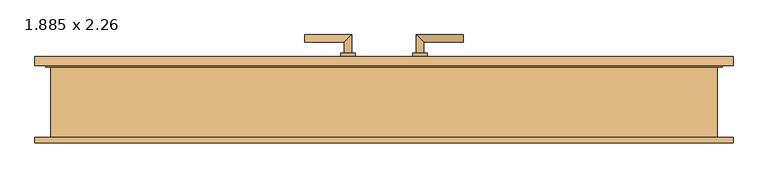
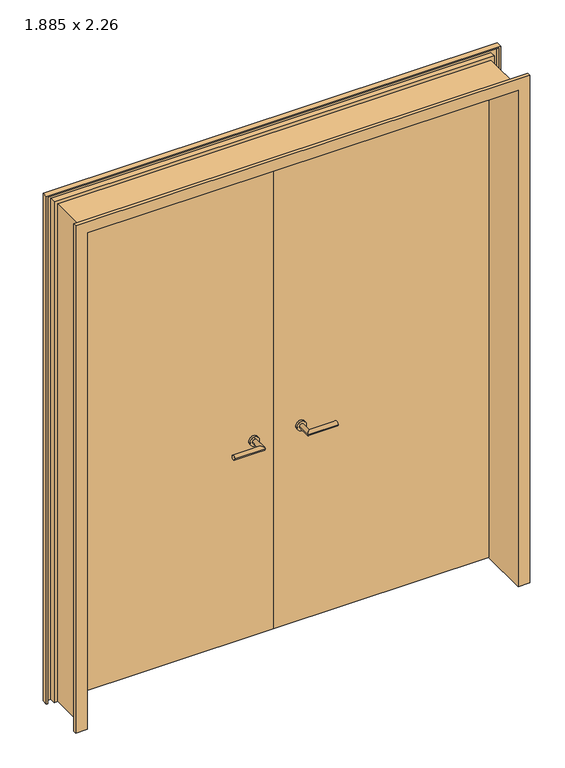
"""IFC4 building model written with IfcOpenShell, lengths in millimetres: door geometry, Drehflügel 2-flg - Stahlzarge : 1.885 x 2.26."""

import ifcopenshell
import ifcopenshell.guid

model = None  # the IFC model being written
_history = None  # IfcOwnerHistory: only IFC2X3 demands one
_inside = {}  # id of a spatial element -> (the spatial element, [elements in it])
_under = {}  # id of a project, library or spatial element -> (it, [spatial elements below it])
_declared = {}  # id of a project -> (the project, [libraries it declares])
_typed = {}  # id of a type object -> (the type object, [elements of that type])
_made_of = {}  # id of a material, layer set ... -> (it, [elements and type objects made of it])


def new_model(schema):
    """Start an empty IFC model of exactly this schema.

    Asked for "IFC4X3", IfcOpenShell would pick the latest addendum, in which some entities
    have other attributes; the version numbers below select the first issue.
    IFC2X3 requires an IfcOwnerHistory on every rooted entity: one is made here for all.
    """
    global model, _history
    if schema == "IFC4X3":
        model = ifcopenshell.file(schema_version=(4, 3, 0, 0))
    else:
        model = ifcopenshell.file(schema=schema)
    _inside.clear()
    _under.clear()
    _declared.clear()
    _typed.clear()
    _made_of.clear()
    _history = None
    if model.schema == "IFC2X3":
        org = make("IfcOrganization", Name="unknown")
        user = make(
            "IfcPersonAndOrganization",
            ThePerson=make("IfcPerson", FamilyName="unknown"),
            TheOrganization=org,
        )
        app = make(
            "IfcApplication",
            ApplicationDeveloper=org,
            Version="unknown",
            ApplicationFullName="unknown",
            ApplicationIdentifier="unknown",
        )
        _history = make(
            "IfcOwnerHistory",
            OwningUser=user,
            OwningApplication=app,
            ChangeAction="ADDED",
            CreationDate=0,
        )
    return model


def make(cls, **values):
    """One entity of the class cls with the attributes given. An attribute that is None is left unset."""
    return model.create_entity(
        cls, **{name: value for name, value in values.items() if value is not None}
    )


def rooted(cls, **values):
    """An entity with a GlobalId (a new one), such as an element, a storey or a relation."""
    return make(cls, GlobalId=ifcopenshell.guid.new(), OwnerHistory=_history, **values)


def si_unit(unit_type, name, prefix=None):
    """IfcSIUnit, for example si_unit("LENGTHUNIT", "METRE", prefix="MILLI")."""
    return make("IfcSIUnit", UnitType=unit_type, Prefix=prefix, Name=name)


def assignment(units):
    """IfcUnitAssignment: the units of a project."""
    return None if units is None else make("IfcUnitAssignment", Units=units)


def point(xyz):
    """IfcCartesianPoint."""
    return None if xyz is None else make("IfcCartesianPoint", Coordinates=xyz)


def direction(xyz):
    """IfcDirection."""
    return None if xyz is None else make("IfcDirection", DirectionRatios=xyz)


def frame(location, z_axis=None, x_axis=None):
    """IfcAxis2Placement3D, a coordinate frame: its origin and axes. An axis left out is left unset."""
    return make(
        "IfcAxis2Placement3D",
        Location=point(location),
        Axis=direction(z_axis),
        RefDirection=direction(x_axis),
    )


def frame_2d(location, x_axis=None):
    """IfcAxis2Placement2D, a coordinate frame in the plane: its origin and x axis."""
    return make(
        "IfcAxis2Placement2D", Location=point(location), RefDirection=direction(x_axis)
    )


def origin():
    """The frame at (0, 0, 0) with its axes left unset."""
    return frame((0.0, 0.0, 0.0))


def origin_with_axes():
    """The frame at (0, 0, 0) with the z axis (0, 0, 1) and the x axis (1, 0, 0) written out."""
    return frame((0.0, 0.0, 0.0), z_axis=(0.0, 0.0, 1.0), x_axis=(1.0, 0.0, 0.0))


def place(relative_to, where):
    """IfcLocalPlacement: puts the frame where relative to a parent placement (None: the world)."""
    return make(
        "IfcLocalPlacement", PlacementRelTo=relative_to, RelativePlacement=where
    )


def context(
    kind, dimensions, precision=None, world=None, true_north=None, identifier=None
):
    """IfcGeometricRepresentationContext, for example the 3D "Model" context."""
    return make(
        "IfcGeometricRepresentationContext",
        ContextIdentifier=identifier,
        ContextType=kind,
        CoordinateSpaceDimension=dimensions,
        Precision=precision,
        WorldCoordinateSystem=world,
        TrueNorth=true_north,
    )


def project(units=None, contexts=None):
    """IfcProject with its units and contexts."""
    return rooted(
        "IfcProject",
        Name="project",
        RepresentationContexts=contexts,
        UnitsInContext=assignment(units),
    )


def spatial(cls, under=None, at=None, **own):
    """A site, building, storey or space (cls), placed at a placement, below another one or the project."""
    s = rooted(cls, ObjectPlacement=at, **own)
    if under is not None:
        _under.setdefault(under.id(), (under, []))[1].append(s)
    return s


def polyline(points):
    """IfcPolyline through the points."""
    return make("IfcPolyline", Points=[point(p) for p in points])


def circle_curve(where, radius):
    """IfcCircle in the frame where."""
    return make("IfcCircle", Position=where, Radius=radius)


def ellipse_curve(where, semi_axis1, semi_axis2):
    """IfcEllipse in the frame where."""
    return make(
        "IfcEllipse", Position=where, SemiAxis1=semi_axis1, SemiAxis2=semi_axis2
    )


def trimmed(basis, trim1, trim2, sense, master):
    """IfcTrimmedCurve: the piece of a basis curve between two trims."""
    return make(
        "IfcTrimmedCurve",
        BasisCurve=basis,
        Trim1=trim1,
        Trim2=trim2,
        SenseAgreement=sense,
        MasterRepresentation=master,
    )


def segment(curve, same_sense, transition):
    """IfcCompositeCurveSegment."""
    return make(
        "IfcCompositeCurveSegment",
        Transition=transition,
        SameSense=same_sense,
        ParentCurve=curve,
    )


def composite_curve(segments, self_intersect=None):
    """IfcCompositeCurve: segments joined end to end."""
    return make("IfcCompositeCurve", Segments=segments, SelfIntersect=self_intersect)


def outline(outer, holes=None, kind="AREA"):
    """IfcArbitraryClosedProfileDef: a profile drawn as a closed curve; with holes, ...WithVoids."""
    if holes is None:
        return make("IfcArbitraryClosedProfileDef", ProfileType=kind, OuterCurve=outer)
    return make(
        "IfcArbitraryProfileDefWithVoids",
        ProfileType=kind,
        OuterCurve=outer,
        InnerCurves=holes,
    )


def extrude(swept, where, along, depth):
    """IfcExtrudedAreaSolid: the profile swept, set in the frame where, extruded along a direction by depth."""
    return make(
        "IfcExtrudedAreaSolid",
        SweptArea=swept,
        Position=where,
        ExtrudedDirection=direction(along),
        Depth=depth,
    )


def faces_of(points, faces, orient=None, outer=None):
    """IfcFace entities. A face is a list of loops; a loop is a list of indices into points, from 0.

    orient and outer hold one flag for each loop. By default every Orientation is true, the
    first loop of a face is its IfcFaceOuterBound and the others are IfcFaceBound.
    """
    made = []
    for i, loops in enumerate(faces):
        bounds = []
        for j, loop in enumerate(loops):
            is_outer = j == 0 if outer is None else outer[i][j]
            bounds.append(
                make(
                    "IfcFaceOuterBound" if is_outer else "IfcFaceBound",
                    Bound=make("IfcPolyLoop", Polygon=[points[k] for k in loop]),
                    Orientation=True if orient is None else orient[i][j],
                )
            )
        made.append(make("IfcFace", Bounds=bounds))
    return made


def faceted_brep(points, faces, orient=None, outer=None, voids=None):
    """IfcFacetedBrep: a solid bounded by flat faces; with voids (closed shells), ...WithVoids."""
    shared = [point(p) for p in points]
    hull = make("IfcClosedShell", CfsFaces=faces_of(shared, faces, orient, outer))
    if voids is None:
        return make("IfcFacetedBrep", Outer=hull)
    return make(
        "IfcFacetedBrepWithVoids",
        Outer=hull,
        Voids=[
            make(cls, CfsFaces=faces_of(shared, fs, o, b)) for cls, fs, o, b in voids
        ],
    )


def shape(context_of_items, identifier, shape_type, items):
    """IfcShapeRepresentation: the items that make up one representation, for example the "Body"."""
    return make(
        "IfcShapeRepresentation",
        ContextOfItems=context_of_items,
        RepresentationIdentifier=identifier,
        RepresentationType=shape_type,
        Items=items,
    )


def source(mapping_origin, context_of_items, identifier, shape_type, items):
    """IfcRepresentationMap: a shape defined once, which mapped items show again and again."""
    return make(
        "IfcRepresentationMap",
        MappingOrigin=mapping_origin,
        MappedRepresentation=shape(context_of_items, identifier, shape_type, items),
    )


def transform(
    local_origin,
    x_axis=None,
    y_axis=None,
    z_axis=None,
    scale=None,
    scale2=None,
    scale3=None,
    uniform=True,
):
    """IfcCartesianTransformationOperator3D, or its non-uniform kind. x_axis, y_axis, z_axis: its Axis1, 2, 3."""
    if uniform:
        return make(
            "IfcCartesianTransformationOperator3D",
            Axis1=direction(x_axis),
            Axis2=direction(y_axis),
            LocalOrigin=point(local_origin),
            Scale=scale,
            Axis3=direction(z_axis),
        )
    return make(
        "IfcCartesianTransformationOperator3DnonUniform",
        Axis1=direction(x_axis),
        Axis2=direction(y_axis),
        LocalOrigin=point(local_origin),
        Scale=scale,
        Axis3=direction(z_axis),
        Scale2=scale2,
        Scale3=scale3,
    )


def mapped(mapping_source, mapping_target):
    """IfcMappedItem: shows the shape of a source again, moved by a transform."""
    return make(
        "IfcMappedItem", MappingSource=mapping_source, MappingTarget=mapping_target
    )


def made_of(thing, what):
    """Note that an element or type object is made of a material, layer set ...; save() writes the relation."""
    if what is not None:
        _made_of.setdefault(what.id(), (what, []))[1].append(thing)
    return thing


def element(
    cls,
    number,
    at=None,
    inside=None,
    cuts=None,
    type_object=None,
    material=None,
    context=None,
    identifier="Body",
    shape_type=None,
    held_by="IfcProductDefinitionShape",
    body=None,
    shapes=None,
    **own,
):
    """One element of the class cls, such as IfcWall. Its Tag is "e" and its number.

    at: its placement. inside: the storey or other place that contains it. cuts: it is an
    opening in that element (IfcRelVoidsElement). A single representation is given by context,
    identifier, shape_type and body (its items); several are given by shapes. held_by: the class
    of the entity that holds the representations. save() writes the other relations.
    """
    e = rooted(cls, Tag="e%d" % number, ObjectPlacement=at, **own)
    if body is not None:
        shapes = [shape(context, identifier, shape_type, body)]
    if shapes is not None:
        e.Representation = make(held_by, Representations=shapes)
    if inside is not None:
        _inside.setdefault(inside.id(), (inside, []))[1].append(e)
    if cuts is not None:
        rooted(
            "IfcRelVoidsElement", RelatingBuildingElement=cuts, RelatedOpeningElement=e
        )
    if type_object is not None:
        _typed.setdefault(type_object.id(), (type_object, []))[1].append(e)
    return made_of(e, material)


def aggregate(whole, parts):
    """IfcRelAggregates: a whole, such as a stair, and the parts it consists of."""
    return rooted("IfcRelAggregates", RelatingObject=whole, RelatedObjects=parts)


def save(model, path):
    """Write the relations noted so far, then the file.

    IfcRelAggregates (storeys below a building ...), IfcRelContainedInSpatialStructure (elements
    in a storey), IfcRelDefinesByType, IfcRelAssociatesMaterial and IfcRelDeclares: one each for
    every whole, place, type object, material and project.
    """
    for whole, parts in _under.values():
        aggregate(whole, parts)
    for where, things in _inside.values():
        rooted(
            "IfcRelContainedInSpatialStructure",
            RelatedElements=things,
            RelatingStructure=where,
        )
    for kind, things in _typed.values():
        rooted("IfcRelDefinesByType", RelatedObjects=things, RelatingType=kind)
    for what, things in _made_of.values():
        rooted("IfcRelAssociatesMaterial", RelatedObjects=things, RelatingMaterial=what)
    for by, libraries in _declared.values():
        rooted("IfcRelDeclares", RelatingContext=by, RelatedDefinitions=libraries)
    model.write(path)


def plane_surface(at):
    """IfcPlane: the flat surface through the origin of the frame at, square to its z axis."""
    return make("IfcPlane", Position=at)


def cylinder_surface(at, radius):
    """IfcCylindricalSurface: all points at the distance radius from the z axis of the frame at."""
    return make("IfcCylindricalSurface", Position=at, Radius=radius)


def advanced_brep(points, edges, surfaces, faces):
    """IfcAdvancedBrep: a solid bounded by faces that lie on surfaces and meet in shared edges.

    An edge is (start, end): straight between two places in points (the first is 0);
    or (start, end, curve); or (start, end, curve, False) where it runs against its curve.
    A face is (place in surfaces, loops), or (place, loops, False) where it looks against
    its surface's normal. A loop lists edges by number (the first is 1), with a minus sign
    where the edge is run from its end to its start. The first loop is the outer one.
    """
    corners = [point(p) for p in points]
    vertices = [make("IfcVertexPoint", VertexGeometry=c) for c in corners]
    made = []
    for start, end, *more in edges:
        made.append(
            make(
                "IfcEdgeCurve",
                EdgeStart=vertices[start],
                EdgeEnd=vertices[end],
                EdgeGeometry=more[0] if more else make("IfcPolyline", Points=[corners[start], corners[end]]),
                SameSense=more[1] if len(more) > 1 else True,
            )
        )
    hull = []
    for where, loops, *sense in faces:
        bounds = []
        for j, loop in enumerate(loops):
            ring = [make("IfcOrientedEdge", EdgeElement=made[abs(k) - 1], Orientation=k > 0) for k in loop]
            bounds.append(
                make(
                    "IfcFaceOuterBound" if j == 0 else "IfcFaceBound",
                    Bound=make("IfcEdgeLoop", EdgeList=ring),
                    Orientation=True,
                )
            )
        hull.append(make("IfcAdvancedFace", Bounds=bounds, FaceSurface=surfaces[where], SameSense=sense[0] if sense else True))
    return make("IfcAdvancedBrep", Outer=make("IfcClosedShell", CfsFaces=hull))


def door_1_885_x_2_26_4807d192(model_context):
    return source(origin(), model_context, "Body", "SolidModel", [
        advanced_brep(
        [(-90.0, 89.4346141, 900.0), (-110.0, 89.4346141, 900.0), (-110.0, 39.4346141, 900.0), (-90.0, 19.4346141, 900.0), (-220.0, 19.4346141, 900.0), (-220.0, 39.4346141, 900.0)],
        [
            (0, 1, circle_curve(frame((-100.0, 89.4346141, 900.0), z_axis=(0.0, 1.0, 0.0), x_axis=(-1.0, 0.0, 0.0)), 10.0)),
            (1, 0, circle_curve(frame((-100.0, 89.4346141, 900.0), z_axis=(0.0, 1.0, 0.0), x_axis=(-1.0, 0.0, 0.0)), 10.0)),
            (1, 2),
            (2, 3, ellipse_curve(frame((-100.0, 29.4346141, 900.0), z_axis=(0.7071067811865385, 0.7071067811865565, 0.0), x_axis=(-0.7071067811865563, 0.7071067811865386, 0.0)), 14.1421356, 10.0)),
            (3, 0),
            (3, 2, ellipse_curve(frame((-100.0, 29.4346141, 900.0), z_axis=(0.7071067811865385, 0.7071067811865565, 0.0), x_axis=(-0.7071067811865563, 0.7071067811865386, 0.0)), 14.1421356, 10.0)),
            (4, 5, circle_curve(frame((-220.0, 29.4346141, 900.0), z_axis=(-1.0, 0.0, 0.0), x_axis=(0.0, 1.0, 0.0)), 10.0)),
            (5, 4, circle_curve(frame((-220.0, 29.4346141, 900.0), z_axis=(-1.0, 0.0, 0.0), x_axis=(0.0, 1.0, 0.0)), 10.0)),
            (2, 5),
            (4, 3),
        ],
        [
            plane_surface(frame((-100.0, 89.4346141, -387.7526403), z_axis=(0.0, 1.0, 0.0), x_axis=(0.0, 0.0, 1.0))),
            cylinder_surface(frame((-100.0, 89.4346141, 900.0), z_axis=(0.0, 1.0, 0.0), x_axis=(-1.0, 0.0, 0.0)), 10.0),
            plane_surface(frame((-220.0, 29.4346141, -387.7526403), z_axis=(-1.0, 0.0, 0.0), x_axis=(0.0, 0.0, 1.0))),
            cylinder_surface(frame((-100.0, 29.4346141, 900.0), z_axis=(1.0, 0.0, 0.0), x_axis=(0.0, 1.0, 0.0)), 10.0),
        ],
        [
            (0, [[1, 2]]),
            (1, [[3, 4, 5, -2]]),
            (1, [[-5, 6, -3, -1]]),
            (2, [[7, 8]]),
            (3, [[9, -7, 10, -4]]),
            (3, [[-10, -8, -9, -6]]),
        ],
    ),
        advanced_brep(
        [(-110.0, 149.4346141, 900.0), (-90.0, 149.4346141, 900.0), (-90.0, 199.4346141, 900.0), (-110.0, 179.4346141, 900.0), (-220.0, 179.4346141, 900.0), (-220.0, 199.4346141, 900.0)],
        [
            (0, 1, circle_curve(frame((-100.0, 149.4346141, 900.0), z_axis=(0.0, -1.0, 0.0), x_axis=(1.0, 0.0, 0.0)), 10.0)),
            (1, 0, circle_curve(frame((-100.0, 149.4346141, 900.0), z_axis=(0.0, -1.0, 0.0), x_axis=(1.0, 0.0, 0.0)), 10.0)),
            (1, 2),
            (2, 3, ellipse_curve(frame((-100.0, 189.4346141, 900.0), z_axis=(0.7071067811865475, -0.7071067811865475, 0.0), x_axis=(-0.7071067811865474, -0.7071067811865476, 0.0)), 14.1421356, 10.0)),
            (3, 0),
            (3, 2, ellipse_curve(frame((-100.0, 189.4346141, 900.0), z_axis=(0.7071067811865475, -0.7071067811865475, 0.0), x_axis=(-0.7071067811865474, -0.7071067811865476, 0.0)), 14.1421356, 10.0)),
            (4, 5, circle_curve(frame((-220.0, 189.4346141, 900.0), z_axis=(-1.0, 0.0, 0.0), x_axis=(0.0, 1.0, 0.0)), 10.0)),
            (5, 4, circle_curve(frame((-220.0, 189.4346141, 900.0), z_axis=(-1.0, 0.0, 0.0), x_axis=(0.0, 1.0, 0.0)), 10.0)),
            (2, 5),
            (4, 3),
        ],
        [
            plane_surface(frame((-100.0, 149.4346141, -387.7526403), z_axis=(0.0, -1.0, 0.0), x_axis=(0.0, 0.0, 1.0))),
            cylinder_surface(frame((-100.0, 149.4346141, 900.0), z_axis=(0.0, -1.0, 0.0), x_axis=(1.0, 0.0, 0.0)), 10.0),
            plane_surface(frame((-220.0, 189.4346141, -387.7526403), z_axis=(-1.0, 0.0, 0.0), x_axis=(0.0, 0.0, 1.0))),
            cylinder_surface(frame((-100.0, 189.4346141, 900.0), z_axis=(1.0, 0.0, 0.0), x_axis=(0.0, 1.0, 0.0)), 10.0),
        ],
        [
            (0, [[1, 2]]),
            (1, [[3, 4, 5, -2]]),
            (1, [[-5, 6, -3, -1]]),
            (2, [[7, 8]]),
            (3, [[9, -7, 10, -4]]),
            (3, [[-10, -8, -9, -6]]),
        ],
    ),
        extrude(outline(composite_curve([segment(trimmed(circle_curve(frame_2d((900.0, -100.0)), 20.0), [point((900.0, -80.0))], [point((900.0, -120.0))], False, "CARTESIAN"), True, "CONTINUOUS"), segment(trimmed(circle_curve(frame_2d((900.0, -100.0)), 20.0), [point((900.0, -120.0))], [point((900.0, -80.0))], False, "CARTESIAN"), True, "CONTINUOUS")], self_intersect=False)), frame((0.0, 79.4346141, 0.0), z_axis=(0.0, 1.0, 0.0), x_axis=(0.0, 0.0, 1.0)), (0.0, 0.0, 1.0), 10.0),
        extrude(outline(composite_curve([segment(trimmed(circle_curve(frame_2d((900.0, -100.0)), 20.0), [point((900.0, -80.0))], [point((900.0, -120.0))], False, "CARTESIAN"), True, "CONTINUOUS"), segment(trimmed(circle_curve(frame_2d((900.0, -100.0)), 20.0), [point((900.0, -120.0))], [point((900.0, -80.0))], False, "CARTESIAN"), True, "CONTINUOUS")], self_intersect=False)), frame((0.0, 139.4346141, 0.0), z_axis=(0.0, 1.0, 0.0), x_axis=(0.0, 0.0, 1.0)), (0.0, 0.0, 1.0), 10.0),
        advanced_brep(
        [(90.0, 89.4346141, 900.0), (110.0, 89.4346141, 900.0), (90.0, 19.4346141, 900.0), (110.0, 39.4346141, 900.0), (220.0, 19.4346141, 900.0), (220.0, 39.4346141, 900.0)],
        [
            (0, 1, circle_curve(frame((100.0, 89.4346141, 900.0), z_axis=(0.0, 1.0, 0.0), x_axis=(1.0, 0.0, 0.0)), 10.0)),
            (1, 0, circle_curve(frame((100.0, 89.4346141, 900.0), z_axis=(0.0, 1.0, 0.0), x_axis=(1.0, 0.0, 0.0)), 10.0)),
            (0, 2),
            (2, 3, ellipse_curve(frame((100.0, 29.4346141, 900.0), z_axis=(-0.7071067811865385, 0.7071067811865565, 0.0), x_axis=(0.7071067811865563, 0.7071067811865386, 0.0)), 14.1421356, 10.0)),
            (3, 1),
            (3, 2, ellipse_curve(frame((100.0, 29.4346141, 900.0), z_axis=(-0.7071067811865385, 0.7071067811865565, 0.0), x_axis=(0.7071067811865563, 0.7071067811865386, 0.0)), 14.1421356, 10.0)),
            (4, 5, circle_curve(frame((220.0, 29.4346141, 900.0), z_axis=(1.0, 0.0, 0.0), x_axis=(0.0, 1.0, 0.0)), 10.0)),
            (5, 4, circle_curve(frame((220.0, 29.4346141, 900.0), z_axis=(1.0, 0.0, 0.0), x_axis=(0.0, 1.0, 0.0)), 10.0)),
            (2, 4),
            (5, 3),
        ],
        [
            plane_surface(frame((100.0, 89.4346141, -387.7526403), z_axis=(0.0, 1.0, 0.0), x_axis=(0.0, 0.0, 1.0))),
            cylinder_surface(frame((100.0, 89.4346141, 900.0), z_axis=(0.0, 1.0, 0.0), x_axis=(1.0, 0.0, 0.0)), 10.0),
            plane_surface(frame((220.0, 29.4346141, -387.7526403), z_axis=(1.0, 0.0, 0.0), x_axis=(0.0, 0.0, 1.0))),
            cylinder_surface(frame((100.0, 29.4346141, 900.0), z_axis=(-1.0, 0.0, 0.0), x_axis=(0.0, 1.0, 0.0)), 10.0),
        ],
        [
            (0, [[1, 2]]),
            (1, [[-1, 3, 4, 5]]),
            (1, [[-2, -5, 6, -3]]),
            (2, [[7, 8]]),
            (3, [[-4, 9, -8, 10]]),
            (3, [[-6, -10, -7, -9]]),
        ],
    ),
        advanced_brep(
        [(110.0, 149.4346141, 900.0), (90.0, 149.4346141, 900.0), (110.0, 179.4346141, 900.0), (90.0, 199.4346141, 900.0), (220.0, 179.4346141, 900.0), (220.0, 199.4346141, 900.0)],
        [
            (0, 1, circle_curve(frame((100.0, 149.4346141, 900.0), z_axis=(0.0, -1.0, 0.0), x_axis=(-1.0, 0.0, 0.0)), 10.0)),
            (1, 0, circle_curve(frame((100.0, 149.4346141, 900.0), z_axis=(0.0, -1.0, 0.0), x_axis=(-1.0, 0.0, 0.0)), 10.0)),
            (0, 2),
            (2, 3, ellipse_curve(frame((100.0, 189.4346141, 900.0), z_axis=(-0.7071067811865475, -0.7071067811865475, 0.0), x_axis=(0.7071067811865474, -0.7071067811865476, 0.0)), 14.1421356, 10.0)),
            (3, 1),
            (3, 2, ellipse_curve(frame((100.0, 189.4346141, 900.0), z_axis=(-0.7071067811865475, -0.7071067811865475, 0.0), x_axis=(0.7071067811865474, -0.7071067811865476, 0.0)), 14.1421356, 10.0)),
            (4, 5, circle_curve(frame((220.0, 189.4346141, 900.0), z_axis=(1.0, 0.0, 0.0), x_axis=(0.0, 1.0, 0.0)), 10.0)),
            (5, 4, circle_curve(frame((220.0, 189.4346141, 900.0), z_axis=(1.0, 0.0, 0.0), x_axis=(0.0, 1.0, 0.0)), 10.0)),
            (2, 4),
            (5, 3),
        ],
        [
            plane_surface(frame((100.0, 149.4346141, -387.7526403), z_axis=(0.0, -1.0, 0.0), x_axis=(0.0, 0.0, 1.0))),
            cylinder_surface(frame((100.0, 149.4346141, 900.0), z_axis=(0.0, -1.0, 0.0), x_axis=(-1.0, 0.0, 0.0)), 10.0),
            plane_surface(frame((220.0, 189.4346141, -387.7526403), z_axis=(1.0, 0.0, 0.0), x_axis=(0.0, 0.0, 1.0))),
            cylinder_surface(frame((100.0, 189.4346141, 900.0), z_axis=(-1.0, 0.0, 0.0), x_axis=(0.0, 1.0, 0.0)), 10.0),
        ],
        [
            (0, [[1, 2]]),
            (1, [[-1, 3, 4, 5]]),
            (1, [[-2, -5, 6, -3]]),
            (2, [[7, 8]]),
            (3, [[-4, 9, -8, 10]]),
            (3, [[-6, -10, -7, -9]]),
        ],
    ),
        extrude(outline(composite_curve([segment(trimmed(circle_curve(frame_2d((900.0, 100.0)), 20.0), [point((900.0, 80.0))], [point((900.0, 120.0))], False, "CARTESIAN"), True, "CONTINUOUS"), segment(trimmed(circle_curve(frame_2d((900.0, 100.0)), 20.0), [point((900.0, 120.0))], [point((900.0, 80.0))], False, "CARTESIAN"), True, "CONTINUOUS")], self_intersect=False)), frame((0.0, 79.4346141, 0.0), z_axis=(0.0, 1.0, 0.0), x_axis=(0.0, 0.0, 1.0)), (0.0, 0.0, 1.0), 10.0),
        extrude(outline(composite_curve([segment(trimmed(circle_curve(frame_2d((900.0, 100.0)), 20.0), [point((900.0, 80.0))], [point((900.0, 120.0))], False, "CARTESIAN"), True, "CONTINUOUS"), segment(trimmed(circle_curve(frame_2d((900.0, 100.0)), 20.0), [point((900.0, 120.0))], [point((900.0, 80.0))], False, "CARTESIAN"), True, "CONTINUOUS")], self_intersect=False)), frame((0.0, 139.4346141, 0.0), z_axis=(0.0, 1.0, 0.0), x_axis=(0.0, 0.0, 1.0)), (0.0, 0.0, 1.0), 10.0),
        extrude(outline(polyline([(0.0, 114.4346141), (-932.5, 114.4346141), (-932.5, 139.4346141), (0.0, 139.4346141), (0.0, 114.4346141)])), origin_with_axes(), (0.0, 0.0, 1.0), 2250.0),
        extrude(outline(polyline([(932.5, 114.4346141), (0.0, 114.4346141), (0.0, 139.4346141), (932.5, 139.4346141), (932.5, 114.4346141)])), origin_with_axes(), (0.0, 0.0, 1.0), 2250.0),
        faceted_brep([(967.0, -100.5653859, 0.0), (917.5, -100.5653859, 0.0), (917.5, 114.4346141, 0.0), (932.5, 114.4346141, 0.0), (932.5, 139.4346141, 0.0), (967.0, 139.4346141, 0.0), (967.0, 114.4346141, 0.0), (962.0, 114.4346141, 0.0), (962.0, 134.4346141, 0.0), (937.5, 134.4346141, 0.0), (937.5, 109.4346141, 0.0), (922.5, 109.4346141, 0.0), (922.5, -95.5653859, 0.0), (962.0, -95.5653859, 0.0), (962.0, -85.5653859, 0.0), (967.0, -85.5653859, 0.0), (967.0, -100.5653859, 2284.5), (-967.0, -100.5653859, 2284.5), (-967.0, -100.5653859, 0.0), (-917.5, -100.5653859, 0.0), (-917.5, -100.5653859, 2235.0), (917.5, -100.5653859, 2235.0), (917.5, 114.4346141, 2235.0), (-917.5, 114.4346141, 2235.0), (-917.5, 114.4346141, 0.0), (-932.5, 114.4346141, 0.0), (-932.5, 114.4346141, 2250.0), (932.5, 114.4346141, 2250.0), (932.5, 139.4346141, 2250.0), (-932.5, 139.4346141, 2250.0), (-932.5, 139.4346141, 0.0), (-967.0, 139.4346141, 0.0), (-967.0, 139.4346141, 2284.5), (967.0, 139.4346141, 2284.5), (967.0, 114.4346141, 2284.5), (-967.0, 114.4346141, 2284.5), (-967.0, 114.4346141, 0.0), (-962.0, 114.4346141, 0.0), (-962.0, 114.4346141, 2279.5), (962.0, 114.4346141, 2279.5), (962.0, 134.4346141, 2279.5), (-962.0, 134.4346141, 2279.5), (-962.0, 134.4346141, 0.0), (-937.5, 134.4346141, 0.0), (-937.5, 134.4346141, 2255.0), (937.5, 134.4346141, 2255.0), (937.5, 109.4346141, 2255.0), (-937.5, 109.4346141, 2255.0), (-937.5, 109.4346141, 0.0), (-922.5, 109.4346141, 0.0), (-922.5, 109.4346141, 2240.0), (922.5, 109.4346141, 2240.0), (922.5, -95.5653859, 2240.0), (-922.5, -95.5653859, 2240.0), (-922.5, -95.5653859, 0.0), (-962.0, -95.5653859, 0.0), (-962.0, -95.5653859, 2279.5), (962.0, -95.5653859, 2279.5), (962.0, -85.5653859, 2279.5), (-962.0, -85.5653859, 2279.5), (-962.0, -85.5653859, 0.0), (-967.0, -85.5653859, 0.0), (-967.0, -85.5653859, 2284.5), (967.0, -85.5653859, 2284.5)], [[[0, 1, 2, 3, 4, 5, 6, 7, 8, 9, 10, 11, 12, 13, 14, 15]], [[1, 0, 16, 17, 18, 19, 20, 21]], [[2, 1, 21, 22]], [[3, 2, 22, 23, 24, 25, 26, 27]], [[4, 3, 27, 28]], [[5, 4, 28, 29, 30, 31, 32, 33]], [[6, 5, 33, 34]], [[7, 6, 34, 35, 36, 37, 38, 39]], [[8, 7, 39, 40]], [[9, 8, 40, 41, 42, 43, 44, 45]], [[10, 9, 45, 46]], [[11, 10, 46, 47, 48, 49, 50, 51]], [[12, 11, 51, 52]], [[13, 12, 52, 53, 54, 55, 56, 57]], [[14, 13, 57, 58]], [[15, 14, 58, 59, 60, 61, 62, 63]], [[0, 15, 63, 16]], [[17, 62, 61, 18]], [[18, 61, 60, 55, 54, 49, 48, 43, 42, 37, 36, 31, 30, 25, 24, 19]], [[23, 20, 19, 24]], [[29, 26, 25, 30]], [[35, 32, 31, 36]], [[41, 38, 37, 42]], [[47, 44, 43, 48]], [[53, 50, 49, 54]], [[59, 56, 55, 60]], [[22, 21, 20, 23]], [[28, 27, 26, 29]], [[34, 33, 32, 35]], [[40, 39, 38, 41]], [[46, 45, 44, 47]], [[52, 51, 50, 53]], [[58, 57, 56, 59]], [[16, 63, 62, 17]]]),
    ])


if __name__ == "__main__":
    model = new_model("IFC4")
    model_context = context("Model", 3, world=origin())
    ifc_project = project(units=[si_unit("LENGTHUNIT", "METRE", prefix="MILLI")], contexts=[model_context])
    site = spatial("IfcSite", under=ifc_project)
    building = spatial("IfcBuilding", under=site)
    placement = place(None, origin())
    door_1_885_x_2_26_shape = door_1_885_x_2_26_4807d192(model_context)
    element("IfcDoor", 1, ObjectType="Drehflügel 2-flg - Stahlzarge : 1.885 x 2.26", at=placement, inside=building, context=model_context, shape_type="MappedRepresentation", body=[
        mapped(door_1_885_x_2_26_shape, transform((0.0, 0.0, 0.0), x_axis=(1.0, 0.0, 0.0), y_axis=(0.0, 1.0, 0.0), z_axis=(0.0, 0.0, 1.0))),
    ])
    save(model, "model.ifc")

# Revit data of these elements
# Type "Drehflügel 2-flg - Stahlzarge : 1.885 x 2.26"
#   Construction Type Id = "MDOOR"
#   Type Mark = "19"
#   Operation = "DoubleDoorSingleSwing"
#   Keynote = "16.03"
#   Analytic Construction = "Metall"
#   Thermal Resistance (R) = 0.270117 (m²·K)/W
#   Heat Transfer Coefficient (U) = 3.7021 W/(m²·K)
#   Rough Width = 1.885 m
#   Rough Height [instance default] = 2.360 m
#   Höhe Türgriff = 0.900 m
#   Height = 2.260 m
#   Fußbodenaufbau [instance default] = 0.100 m
#   Width = 1.885 m
#   Sichtbarkeit Sturzlinien [instance default] = yes
#   Türgriff auswählen [instance default] = element 219327
#   Türgriff [instance default] = none
#   Türflügel [instance default] = none
#   Rahmen/Pfosten [instance default] = Metall - Lackiert - Grau
#   Visual Light Transmittance = 0
#   Solar Heat Gain Coefficient = 0
#   Function = (empty or 0)
#   Wall Closure = (empty or 0)
# Element 1 (IfcDoor, "Drehflügel 2-flg - Stahlzarge : 1.885 x 2.26")
#   Rough Height = 2.260 m
#   Fußbodenaufbau = 0.000 m
#   Materials on its faces: "Metall - Chrom", "Metall - Lackiert - Grau", "Holz - Birke"
# Materials
#   "Metall - Lackiert - Grau": class "Farbe 1", colour RGB 98 98 98, transparency 0, Cost = 0
#   "Metall - Chrom": class "Metall", colour RGB 247 247 247, transparency 0, Cost = 0
#   "Holz - Birke": class "Holz", colour RGB 213 164 103, transparency 0, Cost = 0
